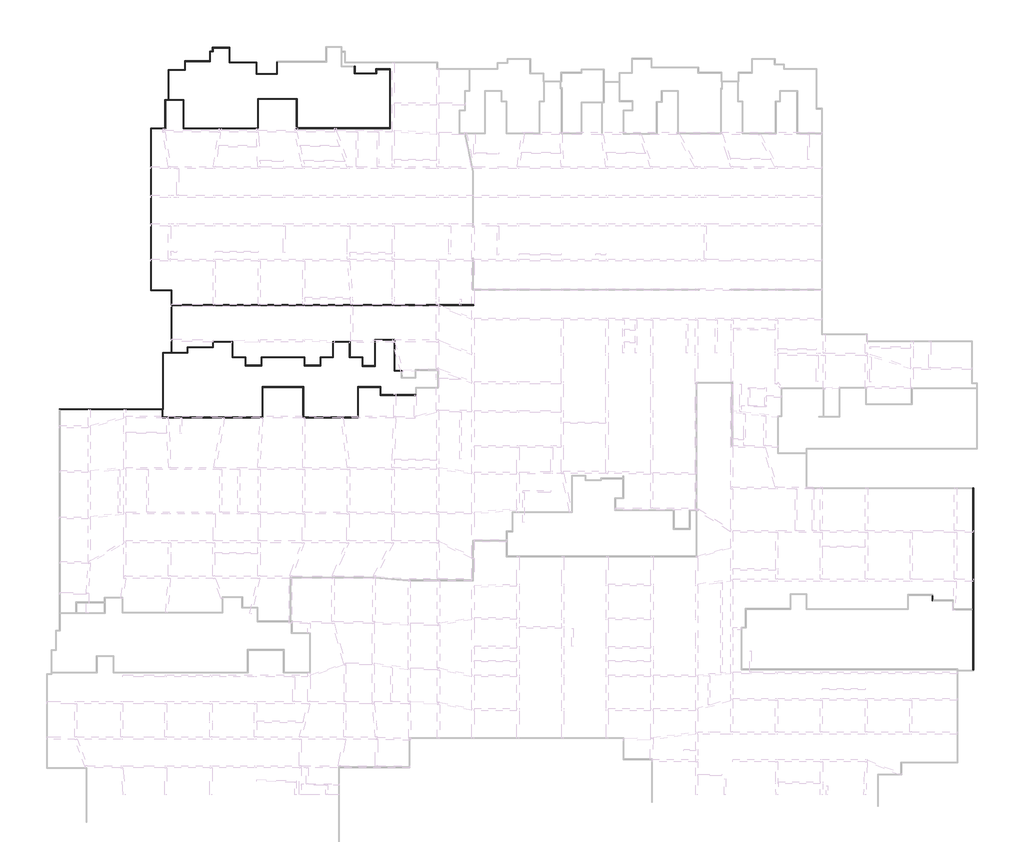
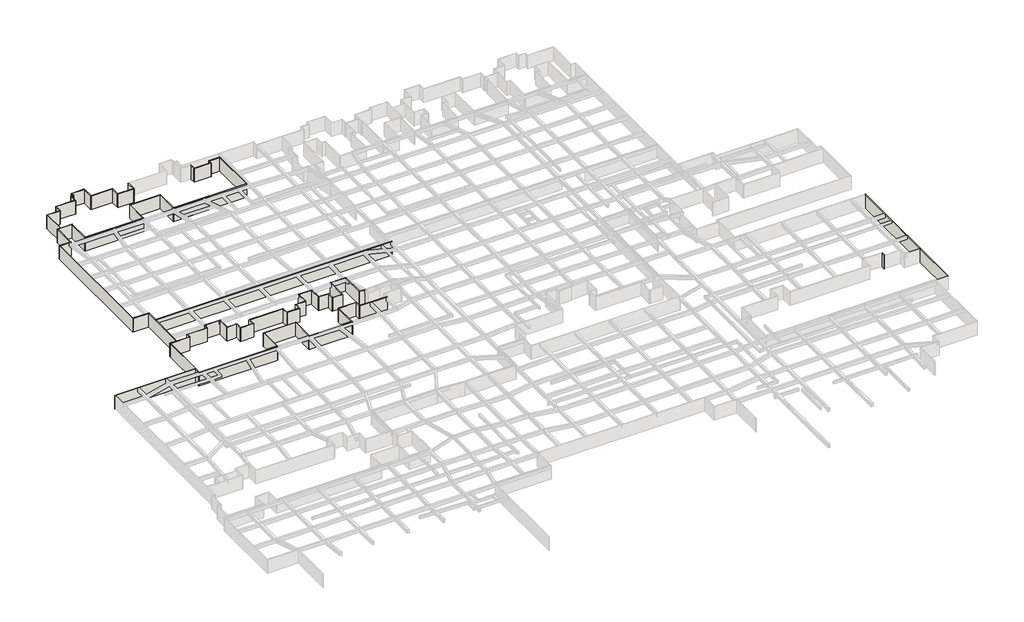
# One storey, part 3 of 16: 70 walls.
"""IFC4 building model written with IfcOpenShell, lengths in millimetres."""

from ifc_helpers import new_model, si_unit, origin, origin_with_axes, place, context, project, spatial, polyline, outline, extrude, faceted_brep, element, save

model = new_model("IFC4")

# Units and contexts
model_context = context("Model", 3, world=origin())
ifc_project = project(units=[si_unit("LENGTHUNIT", "METRE", prefix="MILLI")], contexts=[model_context])

# Site, building, storey
site = spatial("IfcSite", under=ifc_project)
building = spatial("IfcBuilding", under=site)
storey = spatial("IfcBuildingStorey", under=building, Name="户型图", Elevation=0.0)

# Walls
placement = place(None, origin())
element("IfcWall", 1, ObjectType="所有墙体", at=placement, inside=storey, context=model_context, shape_type="Brep", body=[
    faceted_brep([(85783.9765287, 197210.5870026, 0.0), (85663.9765287, 197210.5870026, 0.0), (83068.9386535, 197210.5870026, 0.0), (83068.9386535, 197210.5870026, 3300.0), (85663.9765287, 197210.5870026, 3300.0), (85783.9765287, 197210.5870026, 3300.0), (85783.9765287, 197090.5870026, 0.0), (85783.9765287, 197090.5870026, 3300.0), (83188.9386535, 197090.5870026, 3300.0), (83068.9386535, 197090.5870026, 3300.0), (83068.9386535, 197090.5870026, 0.0), (83188.9386535, 197090.5870026, 0.0)], [[[0, 1, 2, 3, 4, 5]], [[6, 7, 8, 9, 10, 11]], [[2, 1, 0, 6, 11, 10]], [[5, 4, 3, 9, 8, 7]], [[3, 2, 10, 9]], [[0, 5, 7, 6]]]),
])
element("IfcWall", 2, ObjectType="所有墙体", at=placement, inside=storey, context=model_context, shape_type="Brep", body=[
    faceted_brep([(83068.9386535, 197090.5870026, 0.0), (83068.9386535, 167790.5870026, 0.0), (83068.9386535, 167790.5870026, 3300.0), (83068.9386535, 197090.5870026, 3300.0), (83188.9386535, 197090.5870026, 0.0), (83188.9386535, 197090.5870026, 3300.0), (83188.9386535, 167910.5870026, 3300.0), (83188.9386535, 167790.5870026, 3300.0), (83188.9386535, 167790.5870026, 0.0), (83188.9386535, 167910.5870026, 0.0)], [[[0, 1, 2, 3]], [[4, 5, 6, 7, 8, 9]], [[1, 0, 4, 9, 8]], [[3, 2, 7, 6, 5]], [[0, 3, 5, 4]], [[2, 1, 8, 7]]]),
])
element("IfcWall", 3, ObjectType="所有墙体", at=placement, inside=storey, context=model_context, shape_type="Brep", body=[
    faceted_brep([(83188.9386535, 167790.5870026, 0.0), (86768.9386535, 167790.5870026, 0.0), (86888.9386535, 167790.5870026, 0.0), (86888.9386535, 167790.5870026, 3300.0), (86768.9386535, 167790.5870026, 3300.0), (83188.9386535, 167790.5870026, 3300.0), (83188.9386535, 167910.5870026, 0.0), (83188.9386535, 167910.5870026, 3300.0), (86888.9386535, 167910.5870026, 3300.0), (86888.9386535, 167910.5870026, 0.0)], [[[0, 1, 2, 3, 4, 5]], [[6, 7, 8, 9]], [[2, 1, 0, 6, 9]], [[5, 4, 3, 8, 7]], [[0, 5, 7, 6]], [[3, 2, 9, 8]]]),
])
element("IfcWall", 4, ObjectType="所有墙体", at=placement, inside=storey, context=model_context, shape_type="SweptSolid", body=[
    extrude(outline(polyline([(86768.9386535, 156610.5870026), (86768.9386535, 167790.5870026), (86888.9386535, 167790.5870026), (86888.9386535, 156610.5870026), (86768.9386535, 156610.5870026)])), origin_with_axes(), (0.0, 0.0, 1.0), 3300.0),
])
element("IfcWall", 5, ObjectType="所有墙体", at=placement, inside=storey, context=model_context, shape_type="Brep", body=[
    faceted_brep([(89788.9386535, 156610.5870026, 0.0), (89668.9386535, 156610.5870026, 0.0), (86888.9386535, 156610.5870026, 0.0), (86768.9386535, 156610.5870026, 0.0), (85262.5546537, 156610.5870026, 0.0), (85262.5546537, 156610.5870026, 3300.0), (86768.9386535, 156610.5870026, 3300.0), (86888.9386535, 156610.5870026, 3300.0), (89668.9386535, 156610.5870026, 3300.0), (89788.9386535, 156610.5870026, 3300.0), (89788.9386535, 156490.5870026, 0.0), (89788.9386535, 156490.5870026, 3300.0), (85382.5546537, 156490.5870026, 3300.0), (85262.5546537, 156490.5870026, 3300.0), (85262.5546537, 156490.5870026, 0.0), (85382.5546537, 156490.5870026, 0.0)], [[[0, 1, 2, 3, 4, 5, 6, 7, 8, 9]], [[10, 11, 12, 13, 14, 15]], [[4, 3, 2, 1, 0, 10, 15, 14]], [[9, 8, 7, 6, 5, 13, 12, 11]], [[5, 4, 14, 13]], [[0, 9, 11, 10]]]),
])
element("IfcWall", 6, ObjectType="所有墙体", at=placement, inside=storey, context=model_context, shape_type="Brep", body=[
    faceted_brep([(85262.5546537, 156490.5870026, 0.0), (85262.5546537, 146322.3185248, 0.0), (85262.5546537, 146202.3185248, 0.0), (85262.5546537, 146202.3185248, 3300.0), (85262.5546537, 146322.3185248, 3300.0), (85262.5546537, 156490.5870026, 3300.0), (85382.5546537, 156490.5870026, 0.0), (85382.5546537, 156490.5870026, 3300.0), (85382.5546537, 146202.3185248, 3300.0), (85382.5546537, 146202.3185248, 0.0), (85282.4799466, 146202.3185248, 0.0), (85282.4799466, 146202.3185248, 3300.0)], [[[0, 1, 2, 3, 4, 5]], [[6, 7, 8, 9]], [[2, 1, 0, 6, 9, 10]], [[5, 4, 3, 11, 8, 7]], [[0, 5, 7, 6]], [[3, 2, 10, 9, 8, 11]]]),
])
element("IfcWall", 7, ObjectType="所有墙体", at=placement, inside=storey, context=model_context, shape_type="Brep", body=[
    faceted_brep([(85262.5546537, 146322.3185248, 0.0), (66562.5546537, 146322.3185248, 0.0), (66562.5546537, 146322.3185248, 3300.0), (85262.5546537, 146322.3185248, 3300.0), (85262.5546537, 146202.3185248, 0.0), (85262.5546537, 146202.3185248, 3300.0), (85162.4799466, 146202.3185248, 3300.0), (66682.5546537, 146202.3185248, 3300.0), (66562.5546537, 146202.3185248, 3300.0), (66562.5546537, 146202.3185248, 0.0), (66682.5546537, 146202.3185248, 0.0), (85162.4799466, 146202.3185248, 0.0)], [[[0, 1, 2, 3]], [[4, 5, 6, 7, 8, 9, 10, 11]], [[1, 0, 4, 11, 10, 9]], [[3, 2, 8, 7, 6, 5]], [[0, 3, 5, 4]], [[2, 1, 9, 8]]]),
])
element("IfcWall", 8, ObjectType="所有墙体", at=placement, inside=storey, context=model_context, shape_type="Brep", body=[
    faceted_brep([(232107.9308744, 98971.3072201, 0.0), (232107.9308744, 132071.3072201, 0.0), (232107.9308744, 132071.3072201, 3300.0), (232107.9308744, 98971.3072201, 3300.0), (231987.9308744, 98971.3072201, 0.0), (231987.9308744, 98971.3072201, 3300.0), (231987.9308744, 109971.2134701, 3300.0), (231987.9308744, 110091.2134701, 3300.0), (231987.9308744, 131951.3072201, 3300.0), (231987.9308744, 132071.3072201, 3300.0), (231987.9308744, 132071.3072201, 0.0), (231987.9308744, 131951.3072201, 0.0), (231987.9308744, 110091.2134701, 0.0), (231987.9308744, 109971.2134701, 0.0)], [[[0, 1, 2, 3]], [[4, 5, 6, 7, 8, 9, 10, 11, 12, 13]], [[1, 0, 4, 13, 12, 11, 10]], [[3, 2, 9, 8, 7, 6, 5]], [[0, 3, 5, 4]], [[2, 1, 10, 9]]]),
])
element("IfcWall", 9, ObjectType="所有墙体", at=placement, inside=storey, context=model_context, shape_type="Brep", body=[
    faceted_brep([(105913.9765287, 209202.8384701, 0.0), (105913.9765287, 207122.8384701, 0.0), (105913.9765287, 207002.8384701, 0.0), (105913.9765287, 207002.8384701, 3300.0), (105913.9765287, 207122.8384701, 3300.0), (105913.9765287, 209202.8384701, 3300.0), (106033.9765287, 209202.8384701, 0.0), (106033.9765287, 209202.8384701, 3300.0), (106033.9765287, 207002.8384701, 3300.0), (106033.9765287, 207002.8384701, 0.0)], [[[0, 1, 2, 3, 4, 5]], [[6, 7, 8, 9]], [[2, 1, 0, 6, 9]], [[5, 4, 3, 8, 7]], [[0, 5, 7, 6]], [[3, 2, 9, 8]]]),
])
element("IfcWall", 10, ObjectType="所有墙体", at=placement, inside=storey, context=model_context, shape_type="Brep", body=[
    faceted_brep([(105913.9765287, 207122.8384701, 0.0), (102333.9765287, 207122.8384701, 0.0), (102213.9765287, 207122.8384701, 0.0), (102213.9765287, 207122.8384701, 3300.0), (102333.9765287, 207122.8384701, 3300.0), (105913.9765287, 207122.8384701, 3300.0), (105913.9765287, 207002.8384701, 0.0), (105913.9765287, 207002.8384701, 3300.0), (102213.9765287, 207002.8384701, 3300.0), (102213.9765287, 207002.8384701, 0.0)], [[[0, 1, 2, 3, 4, 5]], [[6, 7, 8, 9]], [[2, 1, 0, 6, 9]], [[5, 4, 3, 8, 7]], [[0, 5, 7, 6]], [[3, 2, 9, 8]]]),
])
element("IfcWall", 11, ObjectType="所有墙体", at=placement, inside=storey, context=model_context, shape_type="Brep", body=[
    faceted_brep([(102333.9765287, 207122.8384701, 0.0), (102333.9765287, 209172.8384701, 0.0), (102333.9765287, 209172.8384701, 3300.0), (102333.9765287, 207122.8384701, 3300.0), (102213.9765287, 207122.8384701, 0.0), (102213.9765287, 207122.8384701, 3300.0), (102213.9765287, 209052.8384701, 3300.0), (102213.9765287, 209172.8384701, 3300.0), (102213.9765287, 209172.8384701, 0.0), (102213.9765287, 209052.8384701, 0.0)], [[[0, 1, 2, 3]], [[4, 5, 6, 7, 8, 9]], [[1, 0, 4, 9, 8]], [[3, 2, 7, 6, 5]], [[0, 3, 5, 4]], [[2, 1, 8, 7]]]),
])
element("IfcWall", 12, ObjectType="所有墙体", at=placement, inside=storey, context=model_context, shape_type="Brep", body=[
    faceted_brep([(102213.9765287, 209172.8384701, 0.0), (97383.9765287, 209172.8384701, 0.0), (97263.9765287, 209172.8384701, 0.0), (97263.9765287, 209172.8384701, 3300.0), (97383.9765287, 209172.8384701, 3300.0), (102213.9765287, 209172.8384701, 3300.0), (102213.9765287, 209052.8384701, 0.0), (102213.9765287, 209052.8384701, 3300.0), (97263.9765287, 209052.8384701, 3300.0), (97263.9765287, 209052.8384701, 0.0)], [[[0, 1, 2, 3, 4, 5]], [[6, 7, 8, 9]], [[2, 1, 0, 6, 9]], [[5, 4, 3, 8, 7]], [[0, 5, 7, 6]], [[3, 2, 9, 8]]]),
])
element("IfcWall", 13, ObjectType="所有墙体", at=placement, inside=storey, context=model_context, shape_type="Brep", body=[
    faceted_brep([(97383.9765287, 209172.8384701, 0.0), (97383.9765287, 211872.8384701, 0.0), (97383.9765287, 211872.8384701, 3300.0), (97383.9765287, 209172.8384701, 3300.0), (97263.9765287, 209172.8384701, 0.0), (97263.9765287, 209172.8384701, 3300.0), (97263.9765287, 211752.8384701, 3300.0), (97263.9765287, 211872.8384701, 3300.0), (97263.9765287, 211872.8384701, 0.0), (97263.9765287, 211752.8384701, 0.0)], [[[0, 1, 2, 3]], [[4, 5, 6, 7, 8, 9]], [[1, 0, 4, 9, 8]], [[3, 2, 7, 6, 5]], [[0, 3, 5, 4]], [[2, 1, 8, 7]]]),
])
element("IfcWall", 14, ObjectType="所有墙体", at=placement, inside=storey, context=model_context, shape_type="Brep", body=[
    faceted_brep([(97263.9765287, 211872.8384701, 0.0), (94263.9765287, 211872.8384701, 0.0), (94263.9765287, 211872.8384701, 3300.0), (97263.9765287, 211872.8384701, 3300.0), (97263.9765287, 211752.8384701, 0.0), (97263.9765287, 211752.8384701, 3300.0), (94383.9765287, 211752.8384701, 3300.0), (94263.9765287, 211752.8384701, 3300.0), (94263.9765287, 211752.8384701, 0.0), (94383.9765287, 211752.8384701, 0.0)], [[[0, 1, 2, 3]], [[4, 5, 6, 7, 8, 9]], [[1, 0, 4, 9, 8]], [[3, 2, 7, 6, 5]], [[0, 3, 5, 4]], [[2, 1, 8, 7]]]),
])
element("IfcWall", 15, ObjectType="所有墙体", at=placement, inside=storey, context=model_context, shape_type="Brep", body=[
    faceted_brep([(94263.9765287, 211752.8384701, 0.0), (94263.9765287, 211172.8384701, 0.0), (94263.9765287, 211052.8384701, 0.0), (94263.9765287, 211052.8384701, 3300.0), (94263.9765287, 211172.8384701, 3300.0), (94263.9765287, 211752.8384701, 3300.0), (94383.9765287, 211752.8384701, 0.0), (94383.9765287, 211752.8384701, 3300.0), (94383.9765287, 211052.8384701, 3300.0), (94383.9765287, 211052.8384701, 0.0)], [[[0, 1, 2, 3, 4, 5]], [[6, 7, 8, 9]], [[2, 1, 0, 6, 9]], [[5, 4, 3, 8, 7]], [[0, 5, 7, 6]], [[3, 2, 9, 8]]]),
])
element("IfcWall", 16, ObjectType="所有墙体", at=placement, inside=storey, context=model_context, shape_type="Brep", body=[
    faceted_brep([(94263.9765287, 211172.8384701, 0.0), (93763.9765287, 211172.8384701, 0.0), (93763.9765287, 211172.8384701, 3300.0), (94263.9765287, 211172.8384701, 3300.0), (94263.9765287, 211052.8384701, 0.0), (94263.9765287, 211052.8384701, 3300.0), (93883.9765287, 211052.8384701, 3300.0), (93763.9765287, 211052.8384701, 3300.0), (93763.9765287, 211052.8384701, 0.0), (93883.9765287, 211052.8384701, 0.0)], [[[0, 1, 2, 3]], [[4, 5, 6, 7, 8, 9]], [[1, 0, 4, 9, 8]], [[3, 2, 7, 6, 5]], [[0, 3, 5, 4]], [[2, 1, 8, 7]]]),
])
element("IfcWall", 17, ObjectType="所有墙体", at=placement, inside=storey, context=model_context, shape_type="Brep", body=[
    faceted_brep([(93763.9765287, 211052.8384701, 0.0), (93763.9765287, 209422.8384701, 0.0), (93763.9765287, 209302.8384701, 0.0), (93763.9765287, 209302.8384701, 3300.0), (93763.9765287, 209422.8384701, 3300.0), (93763.9765287, 211052.8384701, 3300.0), (93883.9765287, 211052.8384701, 0.0), (93883.9765287, 211052.8384701, 3300.0), (93883.9765287, 209302.8384701, 3300.0), (93883.9765287, 209302.8384701, 0.0)], [[[0, 1, 2, 3, 4, 5]], [[6, 7, 8, 9]], [[2, 1, 0, 6, 9]], [[5, 4, 3, 8, 7]], [[0, 5, 7, 6]], [[3, 2, 9, 8]]]),
])
element("IfcWall", 18, ObjectType="所有墙体", at=placement, inside=storey, context=model_context, shape_type="Brep", body=[
    faceted_brep([(93763.9765287, 209422.8384701, 0.0), (89263.9765287, 209422.8384701, 0.0), (89263.9765287, 209422.8384701, 3300.0), (93763.9765287, 209422.8384701, 3300.0), (93763.9765287, 209302.8384701, 0.0), (93763.9765287, 209302.8384701, 3300.0), (89383.9765287, 209302.8384701, 3300.0), (89263.9765287, 209302.8384701, 3300.0), (89263.9765287, 209302.8384701, 0.0), (89383.9765287, 209302.8384701, 0.0)], [[[0, 1, 2, 3]], [[4, 5, 6, 7, 8, 9]], [[1, 0, 4, 9, 8]], [[3, 2, 7, 6, 5]], [[0, 3, 5, 4]], [[2, 1, 8, 7]]]),
])
element("IfcWall", 19, ObjectType="所有墙体", at=placement, inside=storey, context=model_context, shape_type="Brep", body=[
    faceted_brep([(89263.9765287, 209302.8384701, 0.0), (89263.9765287, 207822.8384701, 0.0), (89263.9765287, 207702.8384701, 0.0), (89263.9765287, 207702.8384701, 3300.0), (89263.9765287, 207822.8384701, 3300.0), (89263.9765287, 209302.8384701, 3300.0), (89383.9765287, 209302.8384701, 0.0), (89383.9765287, 209302.8384701, 3300.0), (89383.9765287, 207702.8384701, 3300.0), (89383.9765287, 207702.8384701, 0.0)], [[[0, 1, 2, 3, 4, 5]], [[6, 7, 8, 9]], [[2, 1, 0, 6, 9]], [[5, 4, 3, 8, 7]], [[0, 5, 7, 6]], [[3, 2, 9, 8]]]),
])
element("IfcWall", 20, ObjectType="所有墙体", at=placement, inside=storey, context=model_context, shape_type="Brep", body=[
    faceted_brep([(89263.9765287, 207822.8384701, 0.0), (86263.9765287, 207822.8384701, 0.0), (86263.9765287, 207822.8384701, 3300.0), (89263.9765287, 207822.8384701, 3300.0), (89263.9765287, 207702.8384701, 0.0), (89263.9765287, 207702.8384701, 3300.0), (86383.9765287, 207702.8384701, 3300.0), (86263.9765287, 207702.8384701, 3300.0), (86263.9765287, 207702.8384701, 0.0), (86383.9765287, 207702.8384701, 0.0)], [[[0, 1, 2, 3]], [[4, 5, 6, 7, 8, 9]], [[1, 0, 4, 9, 8]], [[3, 2, 7, 6, 5]], [[0, 3, 5, 4]], [[2, 1, 8, 7]]]),
])
element("IfcWall", 21, ObjectType="所有墙体", at=placement, inside=storey, context=model_context, shape_type="SweptSolid", body=[
    extrude(outline(polyline([(86263.9765287, 202422.8384701), (86263.9765287, 207702.8384701), (86383.9765287, 207702.8384701), (86383.9765287, 202422.8384701), (86263.9765287, 202422.8384701)])), origin_with_axes(), (0.0, 0.0, 1.0), 3300.0),
])
element("IfcWall", 22, ObjectType="所有墙体", at=placement, inside=storey, context=model_context, shape_type="Brep", body=[
    faceted_brep([(89083.9765287, 202422.8384701, 0.0), (86383.9765287, 202422.8384701, 0.0), (86263.9765287, 202422.8384701, 0.0), (85663.9765287, 202422.8384701, 0.0), (85663.9765287, 202422.8384701, 3300.0), (86263.9765287, 202422.8384701, 3300.0), (86383.9765287, 202422.8384701, 3300.0), (89083.9765287, 202422.8384701, 3300.0), (89083.9765287, 202302.8384701, 0.0), (89083.9765287, 202302.8384701, 3300.0), (88963.9765287, 202302.8384701, 3300.0), (85783.9765287, 202302.8384701, 3300.0), (85663.9765287, 202302.8384701, 3300.0), (85663.9765287, 202302.8384701, 0.0), (85783.9765287, 202302.8384701, 0.0), (88963.9765287, 202302.8384701, 0.0)], [[[0, 1, 2, 3, 4, 5, 6, 7]], [[8, 9, 10, 11, 12, 13, 14, 15]], [[3, 2, 1, 0, 8, 15, 14, 13]], [[7, 6, 5, 4, 12, 11, 10, 9]], [[4, 3, 13, 12]], [[0, 7, 9, 8]]]),
])
element("IfcWall", 23, ObjectType="所有墙体", at=placement, inside=storey, context=model_context, shape_type="SweptSolid", body=[
    extrude(outline(polyline([(85663.9765287, 197210.5870026), (85663.9765287, 202302.8384701), (85783.9765287, 202302.8384701), (85783.9765287, 197210.5870026), (85663.9765287, 197210.5870026)])), origin_with_axes(), (0.0, 0.0, 1.0), 3300.0),
])
element("IfcWall", 24, ObjectType="所有墙体", at=placement, inside=storey, context=model_context, shape_type="Brep", body=[
    faceted_brep([(88963.9765287, 202302.8384701, 0.0), (88963.9765287, 197102.8384701, 0.0), (88963.9765287, 197102.8384701, 3300.0), (88963.9765287, 202302.8384701, 3300.0), (89083.9765287, 202302.8384701, 0.0), (89083.9765287, 202302.8384701, 3300.0), (89083.9765287, 197222.8384701, 3300.0), (89083.9765287, 197102.8384701, 3300.0), (89083.9765287, 197102.8384701, 0.0), (89083.9765287, 197222.8384701, 0.0)], [[[0, 1, 2, 3]], [[4, 5, 6, 7, 8, 9]], [[1, 0, 4, 9, 8]], [[3, 2, 7, 6, 5]], [[0, 3, 5, 4]], [[2, 1, 8, 7]]]),
])
element("IfcWall", 25, ObjectType="所有墙体", at=placement, inside=storey, context=model_context, shape_type="Brep", body=[
    faceted_brep([(89083.9765287, 197102.8384701, 0.0), (102583.9765287, 197102.8384701, 0.0), (102583.9765287, 197102.8384701, 3300.0), (89083.9765287, 197102.8384701, 3300.0), (89083.9765287, 197222.8384701, 0.0), (89083.9765287, 197222.8384701, 3300.0), (102463.9765287, 197222.8384701, 3300.0), (102583.9765287, 197222.8384701, 3300.0), (102583.9765287, 197222.8384701, 0.0), (102463.9765287, 197222.8384701, 0.0)], [[[0, 1, 2, 3]], [[4, 5, 6, 7, 8, 9]], [[1, 0, 4, 9, 8]], [[3, 2, 7, 6, 5]], [[0, 3, 5, 4]], [[2, 1, 8, 7]]]),
])
element("IfcWall", 26, ObjectType="所有墙体", at=placement, inside=storey, context=model_context, shape_type="Brep", body=[
    faceted_brep([(102583.9765287, 197222.8384701, 0.0), (102583.9765287, 202453.0191342, 0.0), (102583.9765287, 202573.0191342, 0.0), (102583.9765287, 202573.0191342, 3300.0), (102583.9765287, 202453.0191342, 3300.0), (102583.9765287, 197222.8384701, 3300.0), (102463.9765287, 197222.8384701, 0.0), (102463.9765287, 197222.8384701, 3300.0), (102463.9765287, 202573.0191342, 3300.0), (102463.9765287, 202573.0191342, 0.0)], [[[0, 1, 2, 3, 4, 5]], [[6, 7, 8, 9]], [[2, 1, 0, 6, 9]], [[5, 4, 3, 8, 7]], [[0, 5, 7, 6]], [[3, 2, 9, 8]]]),
])
element("IfcWall", 27, ObjectType="所有墙体", at=placement, inside=storey, context=model_context, shape_type="Brep", body=[
    faceted_brep([(102583.9765287, 202453.0191342, 0.0), (109463.9765287, 202453.0191342, 0.0), (109583.9765287, 202453.0191342, 0.0), (109583.9765287, 202453.0191342, 3300.0), (109463.9765287, 202453.0191342, 3300.0), (102583.9765287, 202453.0191342, 3300.0), (102583.9765287, 202573.0191342, 0.0), (102583.9765287, 202573.0191342, 3300.0), (109583.9765287, 202573.0191342, 3300.0), (109583.9765287, 202573.0191342, 0.0)], [[[0, 1, 2, 3, 4, 5]], [[6, 7, 8, 9]], [[2, 1, 0, 6, 9]], [[5, 4, 3, 8, 7]], [[0, 5, 7, 6]], [[3, 2, 9, 8]]]),
])
element("IfcWall", 28, ObjectType="所有墙体", at=placement, inside=storey, context=model_context, shape_type="Brep", body=[
    faceted_brep([(109463.9765287, 202453.0191342, 0.0), (109463.9765287, 197153.0191342, 0.0), (109463.9765287, 197153.0191342, 3300.0), (109463.9765287, 202453.0191342, 3300.0), (109583.9765287, 202453.0191342, 0.0), (109583.9765287, 202453.0191342, 3300.0), (109583.9765287, 197273.0191342, 3300.0), (109583.9765287, 197153.0191342, 3300.0), (109583.9765287, 197153.0191342, 0.0), (109583.9765287, 197273.0191342, 0.0)], [[[0, 1, 2, 3]], [[4, 5, 6, 7, 8, 9]], [[1, 0, 4, 9, 8]], [[3, 2, 7, 6, 5]], [[0, 3, 5, 4]], [[2, 1, 8, 7]]]),
])
element("IfcWall", 29, ObjectType="所有墙体", at=placement, inside=storey, context=model_context, shape_type="Brep", body=[
    faceted_brep([(109583.9765287, 197153.0191342, 0.0), (126483.9765287, 197153.0191342, 0.0), (126483.9765287, 197153.0191342, 3300.0), (109583.9765287, 197153.0191342, 3300.0), (109583.9765287, 197273.0191342, 0.0), (109583.9765287, 197273.0191342, 3300.0), (126363.9765287, 197273.0191342, 3300.0), (126483.9765287, 197273.0191342, 3300.0), (126483.9765287, 197273.0191342, 0.0), (126363.9765287, 197273.0191342, 0.0)], [[[0, 1, 2, 3]], [[4, 5, 6, 7, 8, 9]], [[1, 0, 4, 9, 8]], [[3, 2, 7, 6, 5]], [[0, 3, 5, 4]], [[2, 1, 8, 7]]]),
])
element("IfcWall", 30, ObjectType="所有墙体", at=placement, inside=storey, context=model_context, shape_type="Brep", body=[
    faceted_brep([(126483.9765287, 197273.0191342, 0.0), (126483.9765287, 207973.0191342, 0.0), (126483.9765287, 207973.0191342, 3300.0), (126483.9765287, 197273.0191342, 3300.0), (126363.9765287, 197273.0191342, 0.0), (126363.9765287, 197273.0191342, 3300.0), (126363.9765287, 207853.0191342, 3300.0), (126363.9765287, 207973.0191342, 3300.0), (126363.9765287, 207973.0191342, 0.0), (126363.9765287, 207853.0191342, 0.0)], [[[0, 1, 2, 3]], [[4, 5, 6, 7, 8, 9]], [[1, 0, 4, 9, 8]], [[3, 2, 7, 6, 5]], [[0, 3, 5, 4]], [[2, 1, 8, 7]]]),
])
element("IfcWall", 31, ObjectType="所有墙体", at=placement, inside=storey, context=model_context, shape_type="Brep", body=[
    faceted_brep([(126363.9765287, 207973.0191342, 0.0), (123863.9765287, 207973.0191342, 0.0), (123863.9765287, 207973.0191342, 3300.0), (126363.9765287, 207973.0191342, 3300.0), (126363.9765287, 207853.0191342, 0.0), (126363.9765287, 207853.0191342, 3300.0), (123983.9765287, 207853.0191342, 3300.0), (123863.9765287, 207853.0191342, 3300.0), (123863.9765287, 207853.0191342, 0.0), (123983.9765287, 207853.0191342, 0.0)], [[[0, 1, 2, 3]], [[4, 5, 6, 7, 8, 9]], [[1, 0, 4, 9, 8]], [[3, 2, 7, 6, 5]], [[0, 3, 5, 4]], [[2, 1, 8, 7]]]),
])
element("IfcWall", 32, ObjectType="所有墙体", at=placement, inside=storey, context=model_context, shape_type="Brep", body=[
    faceted_brep([(123863.9765287, 207853.0191342, 0.0), (123863.9765287, 207173.0191342, 0.0), (123863.9765287, 207053.0191342, 0.0), (123863.9765287, 207053.0191342, 3300.0), (123863.9765287, 207173.0191342, 3300.0), (123863.9765287, 207853.0191342, 3300.0), (123983.9765287, 207853.0191342, 0.0), (123983.9765287, 207853.0191342, 3300.0), (123983.9765287, 207053.0191342, 3300.0), (123983.9765287, 207053.0191342, 0.0)], [[[0, 1, 2, 3, 4, 5]], [[6, 7, 8, 9]], [[2, 1, 0, 6, 9]], [[5, 4, 3, 8, 7]], [[0, 5, 7, 6]], [[3, 2, 9, 8]]]),
])
element("IfcWall", 33, ObjectType="所有墙体", at=placement, inside=storey, context=model_context, shape_type="Brep", body=[
    faceted_brep([(123863.9765287, 207173.0191342, 0.0), (120083.9765287, 207173.0191342, 0.0), (119963.9765287, 207173.0191342, 0.0), (119963.9765287, 207173.0191342, 3300.0), (120083.9765287, 207173.0191342, 3300.0), (123863.9765287, 207173.0191342, 3300.0), (123863.9765287, 207053.0191342, 0.0), (123863.9765287, 207053.0191342, 3300.0), (119963.9765287, 207053.0191342, 3300.0), (119963.9765287, 207053.0191342, 0.0)], [[[0, 1, 2, 3, 4, 5]], [[6, 7, 8, 9]], [[2, 1, 0, 6, 9]], [[5, 4, 3, 8, 7]], [[0, 5, 7, 6]], [[3, 2, 9, 8]]]),
])
element("IfcWall", 34, ObjectType="所有墙体", at=placement, inside=storey, context=model_context, shape_type="Brep", body=[
    faceted_brep([(120083.9765287, 207173.0191342, 0.0), (120083.9765287, 208473.0191342, 0.0), (120083.9765287, 208473.0191342, 3300.0), (120083.9765287, 207173.0191342, 3300.0), (119963.9765287, 207173.0191342, 0.0), (119963.9765287, 207173.0191342, 3300.0), (119963.9765287, 208353.0191342, 3300.0), (119963.9765287, 208473.0191342, 3300.0), (119963.9765287, 208473.0191342, 0.0), (119963.9765287, 208353.0191342, 0.0)], [[[0, 1, 2, 3]], [[4, 5, 6, 7, 8, 9]], [[1, 0, 4, 9, 8]], [[3, 2, 7, 6, 5]], [[0, 3, 5, 4]], [[2, 1, 8, 7]]]),
])
element("IfcWall", 35, ObjectType="所有墙体", at=placement, inside=storey, context=model_context, shape_type="SweptSolid", body=[
    extrude(outline(polyline([(86896.2091192, 165222.578939), (141616.2109037, 165222.578939), (141616.2109037, 165102.578939), (86896.2091192, 165102.578939), (86896.2091192, 165222.578939)])), origin_with_axes(), (0.0, 0.0, 1.0), 3300.0),
])
element("IfcWall", 36, ObjectType="所有墙体", at=placement, inside=storey, context=model_context, shape_type="Brep", body=[
    faceted_brep([(89788.9386535, 156610.5870026, 0.0), (89788.9386535, 157474.6509701, 0.0), (89788.9386535, 157594.6509701, 0.0), (89788.9386535, 157594.6509701, 3300.0), (89788.9386535, 157474.6509701, 3300.0), (89788.9386535, 156610.5870026, 3300.0), (89668.9386535, 156610.5870026, 0.0), (89668.9386535, 156610.5870026, 3300.0), (89668.9386535, 157594.6509701, 3300.0), (89668.9386535, 157594.6509701, 0.0)], [[[0, 1, 2, 3, 4, 5]], [[6, 7, 8, 9]], [[2, 1, 0, 6, 9]], [[5, 4, 3, 8, 7]], [[0, 5, 7, 6]], [[3, 2, 9, 8]]]),
])
element("IfcWall", 37, ObjectType="所有墙体", at=placement, inside=storey, context=model_context, shape_type="Brep", body=[
    faceted_brep([(89788.9386535, 157474.6509701, 0.0), (94432.5010488, 157474.6509701, 0.0), (94432.5010488, 157474.6509701, 3300.0), (89788.9386535, 157474.6509701, 3300.0), (89788.9386535, 157594.6509701, 0.0), (89788.9386535, 157594.6509701, 3300.0), (94312.5010488, 157594.6509701, 3300.0), (94432.5010488, 157594.6509701, 3300.0), (94432.5010488, 157594.6509701, 0.0), (94312.5010488, 157594.6509701, 0.0)], [[[0, 1, 2, 3]], [[4, 5, 6, 7, 8, 9]], [[1, 0, 4, 9, 8]], [[3, 2, 7, 6, 5]], [[0, 3, 5, 4]], [[2, 1, 8, 7]]]),
])
element("IfcWall", 38, ObjectType="所有墙体", at=placement, inside=storey, context=model_context, shape_type="Brep", body=[
    faceted_brep([(94432.5010488, 157594.6509701, 0.0), (94432.5010488, 158452.5884701, 0.0), (94432.5010488, 158572.5884701, 0.0), (94432.5010488, 158572.5884701, 3300.0), (94432.5010488, 158452.5884701, 3300.0), (94432.5010488, 157594.6509701, 3300.0), (94312.5010488, 157594.6509701, 0.0), (94312.5010488, 157594.6509701, 3300.0), (94312.5010488, 158572.5884701, 3300.0), (94312.5010488, 158572.5884701, 0.0)], [[[0, 1, 2, 3, 4, 5]], [[6, 7, 8, 9]], [[2, 1, 0, 6, 9]], [[5, 4, 3, 8, 7]], [[0, 5, 7, 6]], [[3, 2, 9, 8]]]),
])
element("IfcWall", 39, ObjectType="所有墙体", at=placement, inside=storey, context=model_context, shape_type="Brep", body=[
    faceted_brep([(94432.5010488, 158452.5884701, 0.0), (97862.4760404, 158452.5884701, 0.0), (97982.4760404, 158452.5884701, 0.0), (97982.4760404, 158452.5884701, 3300.0), (97862.4760404, 158452.5884701, 3300.0), (94432.5010488, 158452.5884701, 3300.0), (94432.5010488, 158572.5884701, 0.0), (94432.5010488, 158572.5884701, 3300.0), (97982.4760404, 158572.5884701, 3300.0), (97982.4760404, 158572.5884701, 0.0)], [[[0, 1, 2, 3, 4, 5]], [[6, 7, 8, 9]], [[2, 1, 0, 6, 9]], [[5, 4, 3, 8, 7]], [[0, 5, 7, 6]], [[3, 2, 9, 8]]]),
])
element("IfcWall", 40, ObjectType="所有墙体", at=placement, inside=storey, context=model_context, shape_type="Brep", body=[
    faceted_brep([(97862.4760404, 158452.5884701, 0.0), (97862.4760404, 155652.5884701, 0.0), (97862.4760404, 155652.5884701, 3300.0), (97862.4760404, 158452.5884701, 3300.0), (97982.4760404, 158452.5884701, 0.0), (97982.4760404, 158452.5884701, 3300.0), (97982.4760404, 155772.5884701, 3300.0), (97982.4760404, 155652.5884701, 3300.0), (97982.4760404, 155652.5884701, 0.0), (97982.4760404, 155772.5884701, 0.0)], [[[0, 1, 2, 3]], [[4, 5, 6, 7, 8, 9]], [[1, 0, 4, 9, 8]], [[3, 2, 7, 6, 5]], [[0, 3, 5, 4]], [[2, 1, 8, 7]]]),
])
element("IfcWall", 41, ObjectType="所有墙体", at=placement, inside=storey, context=model_context, shape_type="Brep", body=[
    faceted_brep([(97982.4760404, 155652.5884701, 0.0), (100162.4760404, 155652.5884701, 0.0), (100282.4760404, 155652.5884701, 0.0), (100282.4760404, 155652.5884701, 3300.0), (100162.4760404, 155652.5884701, 3300.0), (97982.4760404, 155652.5884701, 3300.0), (97982.4760404, 155772.5884701, 0.0), (97982.4760404, 155772.5884701, 3300.0), (100282.4760404, 155772.5884701, 3300.0), (100282.4760404, 155772.5884701, 0.0)], [[[0, 1, 2, 3, 4, 5]], [[6, 7, 8, 9]], [[2, 1, 0, 6, 9]], [[5, 4, 3, 8, 7]], [[0, 5, 7, 6]], [[3, 2, 9, 8]]]),
])
element("IfcWall", 42, ObjectType="所有墙体", at=placement, inside=storey, context=model_context, shape_type="Brep", body=[
    faceted_brep([(100162.4760404, 155652.5884701, 0.0), (100162.4760404, 154152.5884701, 0.0), (100162.4760404, 154152.5884701, 3300.0), (100162.4760404, 155652.5884701, 3300.0), (100282.4760404, 155652.5884701, 0.0), (100282.4760404, 155652.5884701, 3300.0), (100282.4760404, 154272.5884701, 3300.0), (100282.4760404, 154152.5884701, 3300.0), (100282.4760404, 154152.5884701, 0.0), (100282.4760404, 154272.5884701, 0.0)], [[[0, 1, 2, 3]], [[4, 5, 6, 7, 8, 9]], [[1, 0, 4, 9, 8]], [[3, 2, 7, 6, 5]], [[0, 3, 5, 4]], [[2, 1, 8, 7]]]),
])
element("IfcWall", 43, ObjectType="所有墙体", at=placement, inside=storey, context=model_context, shape_type="Brep", body=[
    faceted_brep([(100282.4760404, 154152.5884701, 0.0), (103182.4760404, 154152.5884701, 0.0), (103182.4760404, 154152.5884701, 3300.0), (100282.4760404, 154152.5884701, 3300.0), (100282.4760404, 154272.5884701, 0.0), (100282.4760404, 154272.5884701, 3300.0), (103062.4760404, 154272.5884701, 3300.0), (103182.4760404, 154272.5884701, 3300.0), (103182.4760404, 154272.5884701, 0.0), (103062.4760404, 154272.5884701, 0.0)], [[[0, 1, 2, 3]], [[4, 5, 6, 7, 8, 9]], [[1, 0, 4, 9, 8]], [[3, 2, 7, 6, 5]], [[0, 3, 5, 4]], [[2, 1, 8, 7]]]),
])
element("IfcWall", 44, ObjectType="所有墙体", at=placement, inside=storey, context=model_context, shape_type="Brep", body=[
    faceted_brep([(103182.4760404, 154272.5884701, 0.0), (103182.4760404, 155652.5884701, 0.0), (103182.4760404, 155772.5884701, 0.0), (103182.4760404, 155772.5884701, 3300.0), (103182.4760404, 155652.5884701, 3300.0), (103182.4760404, 154272.5884701, 3300.0), (103062.4760404, 154272.5884701, 0.0), (103062.4760404, 154272.5884701, 3300.0), (103062.4760404, 155772.5884701, 3300.0), (103062.4760404, 155772.5884701, 0.0)], [[[0, 1, 2, 3, 4, 5]], [[6, 7, 8, 9]], [[2, 1, 0, 6, 9]], [[5, 4, 3, 8, 7]], [[0, 5, 7, 6]], [[3, 2, 9, 8]]]),
])
element("IfcWall", 45, ObjectType="所有墙体", at=placement, inside=storey, context=model_context, shape_type="Brep", body=[
    faceted_brep([(103182.4760404, 155652.5884701, 0.0), (110862.4760404, 155652.5884701, 0.0), (110982.4760404, 155652.5884701, 0.0), (110982.4760404, 155652.5884701, 3300.0), (110862.4760404, 155652.5884701, 3300.0), (103182.4760404, 155652.5884701, 3300.0), (103182.4760404, 155772.5884701, 0.0), (103182.4760404, 155772.5884701, 3300.0), (110982.4760404, 155772.5884701, 3300.0), (110982.4760404, 155772.5884701, 0.0)], [[[0, 1, 2, 3, 4, 5]], [[6, 7, 8, 9]], [[2, 1, 0, 6, 9]], [[5, 4, 3, 8, 7]], [[0, 5, 7, 6]], [[3, 2, 9, 8]]]),
])
element("IfcWall", 46, ObjectType="所有墙体", at=placement, inside=storey, context=model_context, shape_type="Brep", body=[
    faceted_brep([(110862.4760404, 155652.5884701, 0.0), (110862.4760404, 154149.6509701, 0.0), (110862.4760404, 154149.6509701, 3300.0), (110862.4760404, 155652.5884701, 3300.0), (110982.4760404, 155652.5884701, 0.0), (110982.4760404, 155652.5884701, 3300.0), (110982.4760404, 154269.6509701, 3300.0), (110982.4760404, 154149.6509701, 3300.0), (110982.4760404, 154149.6509701, 0.0), (110982.4760404, 154269.6509701, 0.0)], [[[0, 1, 2, 3]], [[4, 5, 6, 7, 8, 9]], [[1, 0, 4, 9, 8]], [[3, 2, 7, 6, 5]], [[0, 3, 5, 4]], [[2, 1, 8, 7]]]),
])
element("IfcWall", 47, ObjectType="所有墙体", at=placement, inside=storey, context=model_context, shape_type="Brep", body=[
    faceted_brep([(110982.4760404, 154149.6509701, 0.0), (113882.4760404, 154149.6509701, 0.0), (113882.4760404, 154149.6509701, 3300.0), (110982.4760404, 154149.6509701, 3300.0), (110982.4760404, 154269.6509701, 0.0), (110982.4760404, 154269.6509701, 3300.0), (113762.4760404, 154269.6509701, 3300.0), (113882.4760404, 154269.6509701, 3300.0), (113882.4760404, 154269.6509701, 0.0), (113762.4760404, 154269.6509701, 0.0)], [[[0, 1, 2, 3]], [[4, 5, 6, 7, 8, 9]], [[1, 0, 4, 9, 8]], [[3, 2, 7, 6, 5]], [[0, 3, 5, 4]], [[2, 1, 8, 7]]]),
])
element("IfcWall", 48, ObjectType="所有墙体", at=placement, inside=storey, context=model_context, shape_type="Brep", body=[
    faceted_brep([(113882.4760404, 154269.6509701, 0.0), (113882.4760404, 155652.5884701, 0.0), (113882.4760404, 155772.5884701, 0.0), (113882.4760404, 155772.5884701, 3300.0), (113882.4760404, 155652.5884701, 3300.0), (113882.4760404, 154269.6509701, 3300.0), (113762.4760404, 154269.6509701, 0.0), (113762.4760404, 154269.6509701, 3300.0), (113762.4760404, 155772.5884701, 3300.0), (113762.4760404, 155772.5884701, 0.0)], [[[0, 1, 2, 3, 4, 5]], [[6, 7, 8, 9]], [[2, 1, 0, 6, 9]], [[5, 4, 3, 8, 7]], [[0, 5, 7, 6]], [[3, 2, 9, 8]]]),
])
element("IfcWall", 49, ObjectType="所有墙体", at=placement, inside=storey, context=model_context, shape_type="Brep", body=[
    faceted_brep([(113882.4760404, 155652.5884701, 0.0), (116182.480185, 155652.5884701, 0.0), (116182.480185, 155652.5884701, 3300.0), (113882.4760404, 155652.5884701, 3300.0), (113882.4760404, 155772.5884701, 0.0), (113882.4760404, 155772.5884701, 3300.0), (116062.480185, 155772.5884701, 3300.0), (116182.480185, 155772.5884701, 3300.0), (116182.480185, 155772.5884701, 0.0), (116062.480185, 155772.5884701, 0.0)], [[[0, 1, 2, 3]], [[4, 5, 6, 7, 8, 9]], [[1, 0, 4, 9, 8]], [[3, 2, 7, 6, 5]], [[0, 3, 5, 4]], [[2, 1, 8, 7]]]),
])
element("IfcWall", 50, ObjectType="所有墙体", at=placement, inside=storey, context=model_context, shape_type="Brep", body=[
    faceted_brep([(116182.480185, 155772.5884701, 0.0), (116182.480185, 158452.5884701, 0.0), (116182.480185, 158572.5884701, 0.0), (116182.480185, 158572.5884701, 3300.0), (116182.480185, 158452.5884701, 3300.0), (116182.480185, 155772.5884701, 3300.0), (116062.480185, 155772.5884701, 0.0), (116062.480185, 155772.5884701, 3300.0), (116062.480185, 158572.5884701, 3300.0), (116062.480185, 158572.5884701, 0.0)], [[[0, 1, 2, 3, 4, 5]], [[6, 7, 8, 9]], [[2, 1, 0, 6, 9]], [[5, 4, 3, 8, 7]], [[0, 5, 7, 6]], [[3, 2, 9, 8]]]),
])
element("IfcWall", 51, ObjectType="所有墙体", at=placement, inside=storey, context=model_context, shape_type="Brep", body=[
    faceted_brep([(116182.480185, 158452.5884701, 0.0), (119062.480185, 158452.5884701, 0.0), (119182.480185, 158452.5884701, 0.0), (119182.480185, 158452.5884701, 3300.0), (119062.480185, 158452.5884701, 3300.0), (116182.480185, 158452.5884701, 3300.0), (116182.480185, 158572.5884701, 0.0), (116182.480185, 158572.5884701, 3300.0), (119182.480185, 158572.5884701, 3300.0), (119182.480185, 158572.5884701, 0.0)], [[[0, 1, 2, 3, 4, 5]], [[6, 7, 8, 9]], [[2, 1, 0, 6, 9]], [[5, 4, 3, 8, 7]], [[0, 5, 7, 6]], [[3, 2, 9, 8]]]),
])
element("IfcWall", 52, ObjectType="所有墙体", at=placement, inside=storey, context=model_context, shape_type="Brep", body=[
    faceted_brep([(119062.480185, 158452.5884701, 0.0), (119062.480185, 155652.5884701, 0.0), (119062.480185, 155652.5884701, 3300.0), (119062.480185, 158452.5884701, 3300.0), (119182.480185, 158452.5884701, 0.0), (119182.480185, 158452.5884701, 3300.0), (119182.480185, 155772.5884701, 3300.0), (119182.480185, 155652.5884701, 3300.0), (119182.480185, 155652.5884701, 0.0), (119182.480185, 155772.5884701, 0.0)], [[[0, 1, 2, 3]], [[4, 5, 6, 7, 8, 9]], [[1, 0, 4, 9, 8]], [[3, 2, 7, 6, 5]], [[0, 3, 5, 4]], [[2, 1, 8, 7]]]),
])
element("IfcWall", 53, ObjectType="所有墙体", at=placement, inside=storey, context=model_context, shape_type="Brep", body=[
    faceted_brep([(119182.480185, 155652.5884701, 0.0), (121362.480185, 155652.5884701, 0.0), (121482.480185, 155652.5884701, 0.0), (121482.480185, 155652.5884701, 3300.0), (121362.480185, 155652.5884701, 3300.0), (119182.480185, 155652.5884701, 3300.0), (119182.480185, 155772.5884701, 0.0), (119182.480185, 155772.5884701, 3300.0), (121482.480185, 155772.5884701, 3300.0), (121482.480185, 155772.5884701, 0.0)], [[[0, 1, 2, 3, 4, 5]], [[6, 7, 8, 9]], [[2, 1, 0, 6, 9]], [[5, 4, 3, 8, 7]], [[0, 5, 7, 6]], [[3, 2, 9, 8]]]),
])
element("IfcWall", 54, ObjectType="所有墙体", at=placement, inside=storey, context=model_context, shape_type="Brep", body=[
    faceted_brep([(121362.480185, 155652.5884701, 0.0), (121362.480185, 154052.5884701, 0.0), (121362.480185, 154052.5884701, 3300.0), (121362.480185, 155652.5884701, 3300.0), (121482.480185, 155652.5884701, 0.0), (121482.480185, 155652.5884701, 3300.0), (121482.480185, 154172.5884701, 3300.0), (121482.480185, 154052.5884701, 3300.0), (121482.480185, 154052.5884701, 0.0), (121482.480185, 154172.5884701, 0.0)], [[[0, 1, 2, 3]], [[4, 5, 6, 7, 8, 9]], [[1, 0, 4, 9, 8]], [[3, 2, 7, 6, 5]], [[0, 3, 5, 4]], [[2, 1, 8, 7]]]),
])
element("IfcWall", 55, ObjectType="所有墙体", at=placement, inside=storey, context=model_context, shape_type="Brep", body=[
    faceted_brep([(121482.480185, 154052.5884701, 0.0), (123782.480185, 154052.5884701, 0.0), (123782.480185, 154052.5884701, 3300.0), (121482.480185, 154052.5884701, 3300.0), (121482.480185, 154172.5884701, 0.0), (121482.480185, 154172.5884701, 3300.0), (123662.480185, 154172.5884701, 3300.0), (123782.480185, 154172.5884701, 3300.0), (123782.480185, 154172.5884701, 0.0), (123662.480185, 154172.5884701, 0.0)], [[[0, 1, 2, 3]], [[4, 5, 6, 7, 8, 9]], [[1, 0, 4, 9, 8]], [[3, 2, 7, 6, 5]], [[0, 3, 5, 4]], [[2, 1, 8, 7]]]),
])
element("IfcWall", 56, ObjectType="所有墙体", at=placement, inside=storey, context=model_context, shape_type="Brep", body=[
    faceted_brep([(123782.480185, 154172.5884701, 0.0), (123782.480185, 158825.3546981, 0.0), (123782.480185, 158945.3546981, 0.0), (123782.480185, 158945.3546981, 3300.0), (123782.480185, 158825.3546981, 3300.0), (123782.480185, 154172.5884701, 3300.0), (123662.480185, 154172.5884701, 0.0), (123662.480185, 154172.5884701, 3300.0), (123662.480185, 158945.3546981, 3300.0), (123662.480185, 158945.3546981, 0.0)], [[[0, 1, 2, 3, 4, 5]], [[6, 7, 8, 9]], [[2, 1, 0, 6, 9]], [[5, 4, 3, 8, 7]], [[0, 5, 7, 6]], [[3, 2, 9, 8]]]),
])
element("IfcWall", 57, ObjectType="所有墙体", at=placement, inside=storey, context=model_context, shape_type="Brep", body=[
    faceted_brep([(123782.480185, 158825.3546981, 0.0), (127162.480185, 158825.3546981, 0.0), (127282.480185, 158825.3546981, 0.0), (127282.480185, 158825.3546981, 3300.0), (127162.480185, 158825.3546981, 3300.0), (123782.480185, 158825.3546981, 3300.0), (123782.480185, 158945.3546981, 0.0), (123782.480185, 158945.3546981, 3300.0), (127282.480185, 158945.3546981, 3300.0), (127282.480185, 158945.3546981, 0.0)], [[[0, 1, 2, 3, 4, 5]], [[6, 7, 8, 9]], [[2, 1, 0, 6, 9]], [[5, 4, 3, 8, 7]], [[0, 5, 7, 6]], [[3, 2, 9, 8]]]),
])
element("IfcWall", 58, ObjectType="所有墙体", at=placement, inside=storey, context=model_context, shape_type="Brep", body=[
    faceted_brep([(127162.480185, 158825.3546981, 0.0), (127162.480185, 153225.3546981, 0.0), (127162.480185, 153225.3546981, 3300.0), (127162.480185, 158825.3546981, 3300.0), (127282.480185, 158825.3546981, 0.0), (127282.480185, 158825.3546981, 3300.0), (127282.480185, 153345.3546981, 3300.0), (127282.480185, 153225.3546981, 3300.0), (127282.480185, 153225.3546981, 0.0), (127282.480185, 153345.3546981, 0.0)], [[[0, 1, 2, 3]], [[4, 5, 6, 7, 8, 9]], [[1, 0, 4, 9, 8]], [[3, 2, 7, 6, 5]], [[0, 3, 5, 4]], [[2, 1, 8, 7]]]),
])
element("IfcWall", 59, ObjectType="所有墙体", at=placement, inside=storey, context=model_context, shape_type="Brep", body=[
    faceted_brep([(127282.480185, 153225.3546981, 0.0), (128415.7648004, 153225.3546981, 0.0), (128535.9550541, 153225.3546981, 0.0), (128535.9550541, 153225.3546981, 3300.0), (128415.7648004, 153225.3546981, 3300.0), (127282.480185, 153225.3546981, 3300.0), (127282.480185, 153345.3546981, 0.0), (127282.480185, 153345.3546981, 3300.0), (128529.1950928, 153345.3546981, 3300.0), (128529.1950928, 153345.3546981, 0.0)], [[[0, 1, 2, 3, 4, 5]], [[6, 7, 8, 9]], [[2, 1, 0, 6, 9]], [[5, 4, 3, 8, 7]], [[0, 5, 7, 6]], [[3, 2, 9, 8]]]),
])
element("IfcWall", 60, ObjectType="所有墙体", at=placement, inside=storey, context=model_context, shape_type="Brep", body=[
    faceted_brep([(131062.4799466, 148944.6509701, 0.0), (124782.4799466, 148944.6509701, 0.0), (124662.4799466, 148944.6509701, 0.0), (124662.4799466, 148944.6509701, 3300.0), (124782.4799466, 148944.6509701, 3300.0), (131062.4799466, 148944.6509701, 3300.0), (131062.4799466, 148824.6509701, 0.0), (131062.4799466, 148824.6509701, 3300.0), (124662.4799466, 148824.6509701, 3300.0), (124662.4799466, 148824.6509701, 0.0)], [[[0, 1, 2, 3, 4, 5]], [[6, 7, 8, 9]], [[2, 1, 0, 6, 9]], [[5, 4, 3, 8, 7]], [[0, 5, 7, 6]], [[3, 2, 9, 8]]]),
])
element("IfcWall", 61, ObjectType="所有墙体", at=placement, inside=storey, context=model_context, shape_type="Brep", body=[
    faceted_brep([(124782.4799466, 148944.6509701, 0.0), (124782.4799466, 150369.6509701, 0.0), (124782.4799466, 150369.6509701, 3300.0), (124782.4799466, 148944.6509701, 3300.0), (124662.4799466, 148944.6509701, 0.0), (124662.4799466, 148944.6509701, 3300.0), (124662.4799466, 150249.6509701, 3300.0), (124662.4799466, 150369.6509701, 3300.0), (124662.4799466, 150369.6509701, 0.0), (124662.4799466, 150249.6509701, 0.0)], [[[0, 1, 2, 3]], [[4, 5, 6, 7, 8, 9]], [[1, 0, 4, 9, 8]], [[3, 2, 7, 6, 5]], [[0, 3, 5, 4]], [[2, 1, 8, 7]]]),
])
element("IfcWall", 62, ObjectType="所有墙体", at=placement, inside=storey, context=model_context, shape_type="Brep", body=[
    faceted_brep([(124662.4799466, 150369.6509701, 0.0), (120562.4799466, 150369.6509701, 0.0), (120562.4799466, 150369.6509701, 3300.0), (124662.4799466, 150369.6509701, 3300.0), (124662.4799466, 150249.6509701, 0.0), (124662.4799466, 150249.6509701, 3300.0), (120682.4799466, 150249.6509701, 3300.0), (120562.4799466, 150249.6509701, 3300.0), (120562.4799466, 150249.6509701, 0.0), (120682.4799466, 150249.6509701, 0.0)], [[[0, 1, 2, 3]], [[4, 5, 6, 7, 8, 9]], [[1, 0, 4, 9, 8]], [[3, 2, 7, 6, 5]], [[0, 3, 5, 4]], [[2, 1, 8, 7]]]),
])
element("IfcWall", 63, ObjectType="所有墙体", at=placement, inside=storey, context=model_context, shape_type="Brep", body=[
    faceted_brep([(120562.4799466, 150249.6509701, 0.0), (120562.4799466, 144869.6509701, 0.0), (120562.4799466, 144749.6509701, 0.0), (120562.4799466, 144749.6509701, 3300.0), (120562.4799466, 144869.6509701, 3300.0), (120562.4799466, 150249.6509701, 3300.0), (120682.4799466, 150249.6509701, 0.0), (120682.4799466, 150249.6509701, 3300.0), (120682.4799466, 144749.6509701, 3300.0), (120682.4799466, 144749.6509701, 0.0)], [[[0, 1, 2, 3, 4, 5]], [[6, 7, 8, 9]], [[2, 1, 0, 6, 9]], [[5, 4, 3, 8, 7]], [[0, 5, 7, 6]], [[3, 2, 9, 8]]]),
])
element("IfcWall", 64, ObjectType="所有墙体", at=placement, inside=storey, context=model_context, shape_type="Brep", body=[
    faceted_brep([(120562.4799466, 144869.6509701, 0.0), (110782.4799466, 144869.6509701, 0.0), (110662.4799466, 144869.6509701, 0.0), (110662.4799466, 144869.6509701, 3300.0), (110782.4799466, 144869.6509701, 3300.0), (120562.4799466, 144869.6509701, 3300.0), (120562.4799466, 144749.6509701, 0.0), (120562.4799466, 144749.6509701, 3300.0), (110662.4799466, 144749.6509701, 3300.0), (110662.4799466, 144749.6509701, 0.0)], [[[0, 1, 2, 3, 4, 5]], [[6, 7, 8, 9]], [[2, 1, 0, 6, 9]], [[5, 4, 3, 8, 7]], [[0, 5, 7, 6]], [[3, 2, 9, 8]]]),
])
element("IfcWall", 65, ObjectType="所有墙体", at=placement, inside=storey, context=model_context, shape_type="Brep", body=[
    faceted_brep([(110782.4799466, 144869.6509701, 0.0), (110782.4799466, 150369.6509701, 0.0), (110782.4799466, 150369.6509701, 3300.0), (110782.4799466, 144869.6509701, 3300.0), (110662.4799466, 144869.6509701, 0.0), (110662.4799466, 144869.6509701, 3300.0), (110662.4799466, 150249.6509701, 3300.0), (110662.4799466, 150369.6509701, 3300.0), (110662.4799466, 150369.6509701, 0.0), (110662.4799466, 150249.6509701, 0.0)], [[[0, 1, 2, 3]], [[4, 5, 6, 7, 8, 9]], [[1, 0, 4, 9, 8]], [[3, 2, 7, 6, 5]], [[0, 3, 5, 4]], [[2, 1, 8, 7]]]),
])
element("IfcWall", 66, ObjectType="所有墙体", at=placement, inside=storey, context=model_context, shape_type="Brep", body=[
    faceted_brep([(110662.4799466, 150369.6509701, 0.0), (103262.4799466, 150369.6509701, 0.0), (103262.4799466, 150369.6509701, 3300.0), (110662.4799466, 150369.6509701, 3300.0), (110662.4799466, 150249.6509701, 0.0), (110662.4799466, 150249.6509701, 3300.0), (103382.4799466, 150249.6509701, 3300.0), (103262.4799466, 150249.6509701, 3300.0), (103262.4799466, 150249.6509701, 0.0), (103382.4799466, 150249.6509701, 0.0)], [[[0, 1, 2, 3]], [[4, 5, 6, 7, 8, 9]], [[1, 0, 4, 9, 8]], [[3, 2, 7, 6, 5]], [[0, 3, 5, 4]], [[2, 1, 8, 7]]]),
])
element("IfcWall", 67, ObjectType="所有墙体", at=placement, inside=storey, context=model_context, shape_type="Brep", body=[
    faceted_brep([(103262.4799466, 150249.6509701, 0.0), (103262.4799466, 144869.6509701, 0.0), (103262.4799466, 144749.6509701, 0.0), (103262.4799466, 144749.6509701, 3300.0), (103262.4799466, 144869.6509701, 3300.0), (103262.4799466, 150249.6509701, 3300.0), (103382.4799466, 150249.6509701, 0.0), (103382.4799466, 150249.6509701, 3300.0), (103382.4799466, 144749.6509701, 3300.0), (103382.4799466, 144749.6509701, 0.0)], [[[0, 1, 2, 3, 4, 5]], [[6, 7, 8, 9]], [[2, 1, 0, 6, 9]], [[5, 4, 3, 8, 7]], [[0, 5, 7, 6]], [[3, 2, 9, 8]]]),
])
element("IfcWall", 68, ObjectType="所有墙体", at=placement, inside=storey, context=model_context, shape_type="Brep", body=[
    faceted_brep([(103262.4799466, 144869.6509701, 0.0), (85282.4799466, 144869.6509701, 0.0), (85162.4799466, 144869.6509701, 0.0), (85162.4799466, 144869.6509701, 3300.0), (85282.4799466, 144869.6509701, 3300.0), (103262.4799466, 144869.6509701, 3300.0), (103262.4799466, 144749.6509701, 0.0), (103262.4799466, 144749.6509701, 3300.0), (85162.4799466, 144749.6509701, 3300.0), (85162.4799466, 144749.6509701, 0.0)], [[[0, 1, 2, 3, 4, 5]], [[6, 7, 8, 9]], [[2, 1, 0, 6, 9]], [[5, 4, 3, 8, 7]], [[0, 5, 7, 6]], [[3, 2, 9, 8]]]),
])
element("IfcWall", 69, ObjectType="所有墙体", at=placement, inside=storey, context=model_context, shape_type="Brep", body=[
    faceted_brep([(85282.4799466, 144869.6509701, 0.0), (85282.4799466, 146202.3185248, 0.0), (85282.4799466, 146202.3185248, 3300.0), (85282.4799466, 144869.6509701, 3300.0), (85162.4799466, 144869.6509701, 0.0), (85162.4799466, 144869.6509701, 3300.0), (85162.4799466, 146202.3185248, 3300.0), (85162.4799466, 146202.3185248, 0.0), (85262.5546537, 146202.3185248, 0.0), (85262.5546537, 146202.3185248, 3300.0)], [[[0, 1, 2, 3]], [[4, 5, 6, 7]], [[1, 0, 4, 7, 8]], [[3, 2, 9, 6, 5]], [[0, 3, 5, 4]], [[2, 1, 8, 7, 6, 9]]]),
])
element("IfcWall", 70, ObjectType="所有墙体", at=placement, inside=storey, context=model_context, shape_type="Brep", body=[
    faceted_brep([(224612.920801, 112601.2124935, 0.0), (224612.920801, 111591.2134701, 0.0), (224612.920801, 111591.2134701, 3300.0), (224612.920801, 112601.2124935, 3300.0), (224732.920801, 112601.2124935, 0.0), (224732.920801, 112601.2124935, 3300.0), (224732.920801, 111711.2134701, 3300.0), (224732.920801, 111591.2134701, 3300.0), (224732.920801, 111591.2134701, 0.0), (224732.920801, 111711.2134701, 0.0)], [[[0, 1, 2, 3]], [[4, 5, 6, 7, 8, 9]], [[1, 0, 4, 9, 8]], [[3, 2, 7, 6, 5]], [[0, 3, 5, 4]], [[2, 1, 8, 7]]]),
])

save(model, "model.ifc")

# Revit data of these elements
# Type "所有墙体"
#   Layers, outside or top first: 120 mm "默认" (function 1)
# Elements 1, 2, 3, 4, 5, 6, 7, 8, 9, 10, 11, 12, 13, 14, 15, 16, 17, 18, 19, 20, 21, 22, 23, 24, 25, 26, 27, 28, 29, 30, 31, 32, 33, 34, 35, 36, 37, 38, 39, 40, 41, 42, 43, 44, 45, 46, 47, 48, 49, 50, 51, 52, 53, 54, 55, 56, 57, 58, 59, 60, 61, 62, 63, 64, 65, 66, 67, 68, 69, 70 (IfcWall, "所有墙体")
#   Top Offset = 0 mm
#   Base Offset = 0 mm
#   wall height = 3300 mm
#   Phase Created = 新构造
#   Base Constraint = 户型图
#   Top Constraint = 层高
#   Materials on its faces: "默认"
# Materials
#   "默认": class "其他", colour RGB 192 192 192, transparency 0, Cost = 0
